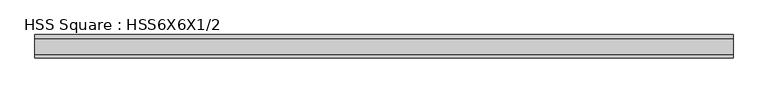
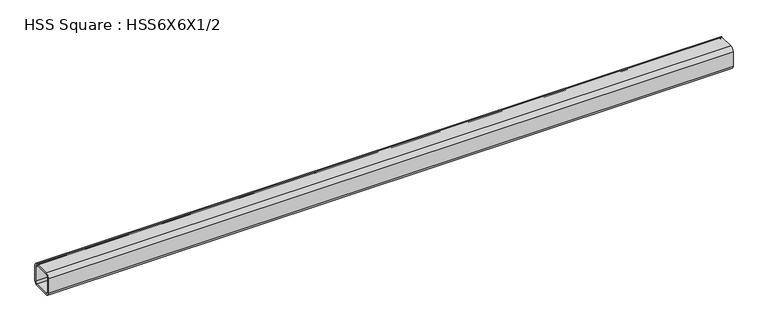
"""IFC4 building model written with IfcOpenShell, lengths in millimetres: member geometry, HSS Square : HSS6X6X1/2."""

import ifcopenshell
import ifcopenshell.guid

model = None  # the IFC model being written
_history = None  # IfcOwnerHistory: only IFC2X3 demands one
_inside = {}  # id of a spatial element -> (the spatial element, [elements in it])
_under = {}  # id of a project, library or spatial element -> (it, [spatial elements below it])
_declared = {}  # id of a project -> (the project, [libraries it declares])
_typed = {}  # id of a type object -> (the type object, [elements of that type])
_made_of = {}  # id of a material, layer set ... -> (it, [elements and type objects made of it])


def new_model(schema):
    """Start an empty IFC model of exactly this schema.

    Asked for "IFC4X3", IfcOpenShell would pick the latest addendum, in which some entities
    have other attributes; the version numbers below select the first issue.
    IFC2X3 requires an IfcOwnerHistory on every rooted entity: one is made here for all.
    """
    global model, _history
    if schema == "IFC4X3":
        model = ifcopenshell.file(schema_version=(4, 3, 0, 0))
    else:
        model = ifcopenshell.file(schema=schema)
    _inside.clear()
    _under.clear()
    _declared.clear()
    _typed.clear()
    _made_of.clear()
    _history = None
    if model.schema == "IFC2X3":
        org = make("IfcOrganization", Name="unknown")
        user = make(
            "IfcPersonAndOrganization",
            ThePerson=make("IfcPerson", FamilyName="unknown"),
            TheOrganization=org,
        )
        app = make(
            "IfcApplication",
            ApplicationDeveloper=org,
            Version="unknown",
            ApplicationFullName="unknown",
            ApplicationIdentifier="unknown",
        )
        _history = make(
            "IfcOwnerHistory",
            OwningUser=user,
            OwningApplication=app,
            ChangeAction="ADDED",
            CreationDate=0,
        )
    return model


def make(cls, **values):
    """One entity of the class cls with the attributes given. An attribute that is None is left unset."""
    return model.create_entity(
        cls, **{name: value for name, value in values.items() if value is not None}
    )


def rooted(cls, **values):
    """An entity with a GlobalId (a new one), such as an element, a storey or a relation."""
    return make(cls, GlobalId=ifcopenshell.guid.new(), OwnerHistory=_history, **values)


def si_unit(unit_type, name, prefix=None):
    """IfcSIUnit, for example si_unit("LENGTHUNIT", "METRE", prefix="MILLI")."""
    return make("IfcSIUnit", UnitType=unit_type, Prefix=prefix, Name=name)


def assignment(units):
    """IfcUnitAssignment: the units of a project."""
    return None if units is None else make("IfcUnitAssignment", Units=units)


def point(xyz):
    """IfcCartesianPoint."""
    return None if xyz is None else make("IfcCartesianPoint", Coordinates=xyz)


def direction(xyz):
    """IfcDirection."""
    return None if xyz is None else make("IfcDirection", DirectionRatios=xyz)


def frame(location, z_axis=None, x_axis=None):
    """IfcAxis2Placement3D, a coordinate frame: its origin and axes. An axis left out is left unset."""
    return make(
        "IfcAxis2Placement3D",
        Location=point(location),
        Axis=direction(z_axis),
        RefDirection=direction(x_axis),
    )


def frame_2d(location, x_axis=None):
    """IfcAxis2Placement2D, a coordinate frame in the plane: its origin and x axis."""
    return make(
        "IfcAxis2Placement2D", Location=point(location), RefDirection=direction(x_axis)
    )


def origin():
    """The frame at (0, 0, 0) with its axes left unset."""
    return frame((0.0, 0.0, 0.0))


def place(relative_to, where):
    """IfcLocalPlacement: puts the frame where relative to a parent placement (None: the world)."""
    return make(
        "IfcLocalPlacement", PlacementRelTo=relative_to, RelativePlacement=where
    )


def context(
    kind, dimensions, precision=None, world=None, true_north=None, identifier=None
):
    """IfcGeometricRepresentationContext, for example the 3D "Model" context."""
    return make(
        "IfcGeometricRepresentationContext",
        ContextIdentifier=identifier,
        ContextType=kind,
        CoordinateSpaceDimension=dimensions,
        Precision=precision,
        WorldCoordinateSystem=world,
        TrueNorth=true_north,
    )


def project(units=None, contexts=None):
    """IfcProject with its units and contexts."""
    return rooted(
        "IfcProject",
        Name="project",
        RepresentationContexts=contexts,
        UnitsInContext=assignment(units),
    )


def spatial(cls, under=None, at=None, **own):
    """A site, building, storey or space (cls), placed at a placement, below another one or the project."""
    s = rooted(cls, ObjectPlacement=at, **own)
    if under is not None:
        _under.setdefault(under.id(), (under, []))[1].append(s)
    return s


def polyline(points):
    """IfcPolyline through the points."""
    return make("IfcPolyline", Points=[point(p) for p in points])


def circle_curve(where, radius):
    """IfcCircle in the frame where."""
    return make("IfcCircle", Position=where, Radius=radius)


def trimmed(basis, trim1, trim2, sense, master):
    """IfcTrimmedCurve: the piece of a basis curve between two trims."""
    return make(
        "IfcTrimmedCurve",
        BasisCurve=basis,
        Trim1=trim1,
        Trim2=trim2,
        SenseAgreement=sense,
        MasterRepresentation=master,
    )


def segment(curve, same_sense, transition):
    """IfcCompositeCurveSegment."""
    return make(
        "IfcCompositeCurveSegment",
        Transition=transition,
        SameSense=same_sense,
        ParentCurve=curve,
    )


def composite_curve(segments, self_intersect=None):
    """IfcCompositeCurve: segments joined end to end."""
    return make("IfcCompositeCurve", Segments=segments, SelfIntersect=self_intersect)


def outline(outer, holes=None, kind="AREA"):
    """IfcArbitraryClosedProfileDef: a profile drawn as a closed curve; with holes, ...WithVoids."""
    if holes is None:
        return make("IfcArbitraryClosedProfileDef", ProfileType=kind, OuterCurve=outer)
    return make(
        "IfcArbitraryProfileDefWithVoids",
        ProfileType=kind,
        OuterCurve=outer,
        InnerCurves=holes,
    )


def extrude(swept, where, along, depth):
    """IfcExtrudedAreaSolid: the profile swept, set in the frame where, extruded along a direction by depth."""
    return make(
        "IfcExtrudedAreaSolid",
        SweptArea=swept,
        Position=where,
        ExtrudedDirection=direction(along),
        Depth=depth,
    )


def shape(context_of_items, identifier, shape_type, items):
    """IfcShapeRepresentation: the items that make up one representation, for example the "Body"."""
    return make(
        "IfcShapeRepresentation",
        ContextOfItems=context_of_items,
        RepresentationIdentifier=identifier,
        RepresentationType=shape_type,
        Items=items,
    )


def source(mapping_origin, context_of_items, identifier, shape_type, items):
    """IfcRepresentationMap: a shape defined once, which mapped items show again and again."""
    return make(
        "IfcRepresentationMap",
        MappingOrigin=mapping_origin,
        MappedRepresentation=shape(context_of_items, identifier, shape_type, items),
    )


def transform(
    local_origin,
    x_axis=None,
    y_axis=None,
    z_axis=None,
    scale=None,
    scale2=None,
    scale3=None,
    uniform=True,
):
    """IfcCartesianTransformationOperator3D, or its non-uniform kind. x_axis, y_axis, z_axis: its Axis1, 2, 3."""
    if uniform:
        return make(
            "IfcCartesianTransformationOperator3D",
            Axis1=direction(x_axis),
            Axis2=direction(y_axis),
            LocalOrigin=point(local_origin),
            Scale=scale,
            Axis3=direction(z_axis),
        )
    return make(
        "IfcCartesianTransformationOperator3DnonUniform",
        Axis1=direction(x_axis),
        Axis2=direction(y_axis),
        LocalOrigin=point(local_origin),
        Scale=scale,
        Axis3=direction(z_axis),
        Scale2=scale2,
        Scale3=scale3,
    )


def mapped(mapping_source, mapping_target):
    """IfcMappedItem: shows the shape of a source again, moved by a transform."""
    return make(
        "IfcMappedItem", MappingSource=mapping_source, MappingTarget=mapping_target
    )


def made_of(thing, what):
    """Note that an element or type object is made of a material, layer set ...; save() writes the relation."""
    if what is not None:
        _made_of.setdefault(what.id(), (what, []))[1].append(thing)
    return thing


def element(
    cls,
    number,
    at=None,
    inside=None,
    cuts=None,
    type_object=None,
    material=None,
    context=None,
    identifier="Body",
    shape_type=None,
    held_by="IfcProductDefinitionShape",
    body=None,
    shapes=None,
    **own,
):
    """One element of the class cls, such as IfcWall. Its Tag is "e" and its number.

    at: its placement. inside: the storey or other place that contains it. cuts: it is an
    opening in that element (IfcRelVoidsElement). A single representation is given by context,
    identifier, shape_type and body (its items); several are given by shapes. held_by: the class
    of the entity that holds the representations. save() writes the other relations.
    """
    e = rooted(cls, Tag="e%d" % number, ObjectPlacement=at, **own)
    if body is not None:
        shapes = [shape(context, identifier, shape_type, body)]
    if shapes is not None:
        e.Representation = make(held_by, Representations=shapes)
    if inside is not None:
        _inside.setdefault(inside.id(), (inside, []))[1].append(e)
    if cuts is not None:
        rooted(
            "IfcRelVoidsElement", RelatingBuildingElement=cuts, RelatedOpeningElement=e
        )
    if type_object is not None:
        _typed.setdefault(type_object.id(), (type_object, []))[1].append(e)
    return made_of(e, material)


def aggregate(whole, parts):
    """IfcRelAggregates: a whole, such as a stair, and the parts it consists of."""
    return rooted("IfcRelAggregates", RelatingObject=whole, RelatedObjects=parts)


def save(model, path):
    """Write the relations noted so far, then the file.

    IfcRelAggregates (storeys below a building ...), IfcRelContainedInSpatialStructure (elements
    in a storey), IfcRelDefinesByType, IfcRelAssociatesMaterial and IfcRelDeclares: one each for
    every whole, place, type object, material and project.
    """
    for whole, parts in _under.values():
        aggregate(whole, parts)
    for where, things in _inside.values():
        rooted(
            "IfcRelContainedInSpatialStructure",
            RelatedElements=things,
            RelatingStructure=where,
        )
    for kind, things in _typed.values():
        rooted("IfcRelDefinesByType", RelatedObjects=things, RelatingType=kind)
    for what, things in _made_of.values():
        rooted("IfcRelAssociatesMaterial", RelatedObjects=things, RelatingMaterial=what)
    for by, libraries in _declared.values():
        rooted("IfcRelDeclares", RelatingContext=by, RelatedDefinitions=libraries)
    model.write(path)


def hss_square_hss6x6x1_2_15cbbfaa(model_context):
    return source(origin(), model_context, "Body", "SweptSolid", [
        extrude(outline(composite_curve([segment(polyline([(76.2, 50.8), (76.2, -50.8)]), True, "CONTINUOUS"), segment(trimmed(circle_curve(frame_2d((50.8, -50.8)), 25.4), [point((76.2, -50.8))], [point((50.8, -76.2))], False, "CARTESIAN"), True, "CONTINUOUS"), segment(polyline([(50.8, -76.2), (-50.8, -76.2)]), True, "CONTINUOUS"), segment(trimmed(circle_curve(frame_2d((-50.8, -50.8)), 25.4), [point((-50.8, -76.2))], [point((-76.2, -50.8))], False, "CARTESIAN"), True, "CONTINUOUS"), segment(polyline([(-76.2, -50.8), (-76.2, 50.8)]), True, "CONTINUOUS"), segment(trimmed(circle_curve(frame_2d((-50.8, 50.8)), 25.4), [point((-76.2, 50.8))], [point((-50.8, 76.2))], False, "CARTESIAN"), True, "CONTINUOUS"), segment(polyline([(-50.8, 76.2), (50.8, 76.2)]), True, "CONTINUOUS"), segment(trimmed(circle_curve(frame_2d((50.8, 50.8)), 25.4), [point((50.8, 76.2))], [point((76.2, 50.8))], False, "CARTESIAN"), True, "CONTINUOUS")], self_intersect=False), holes=[composite_curve([segment(trimmed(circle_curve(frame_2d((-50.8, 50.8)), 12.7), [point((-50.8, 63.5))], [point((-63.5, 50.8))], True, "CARTESIAN"), True, "CONTINUOUS"), segment(polyline([(-63.5, 50.8), (-63.5, -50.8)]), True, "CONTINUOUS"), segment(trimmed(circle_curve(frame_2d((-50.8, -50.8)), 12.7), [point((-63.5, -50.8))], [point((-50.8, -63.5))], True, "CARTESIAN"), True, "CONTINUOUS"), segment(polyline([(-50.8, -63.5), (50.8, -63.5)]), True, "CONTINUOUS"), segment(trimmed(circle_curve(frame_2d((50.8, -50.8)), 12.7), [point((50.8, -63.5))], [point((63.5, -50.8))], True, "CARTESIAN"), True, "CONTINUOUS"), segment(polyline([(63.5, -50.8), (63.5, 50.8)]), True, "CONTINUOUS"), segment(trimmed(circle_curve(frame_2d((50.8, 50.8)), 12.7), [point((63.5, 50.8))], [point((50.8, 63.5))], True, "CARTESIAN"), True, "CONTINUOUS"), segment(polyline([(50.8, 63.5), (-50.8, 63.5)]), True, "CONTINUOUS")], self_intersect=False)]), frame((-2104.169756, 0.0, 0.0), z_axis=(1.0, 0.0, 0.0), x_axis=(0.0, 1.0, 0.0)), (0.0, 0.0, 1.0), 4524.6444945),
    ])


if __name__ == "__main__":
    model = new_model("IFC4")
    model_context = context("Model", 3, world=origin())
    ifc_project = project(units=[si_unit("LENGTHUNIT", "METRE", prefix="MILLI")], contexts=[model_context])
    site = spatial("IfcSite", under=ifc_project)
    building = spatial("IfcBuilding", under=site)
    placement = place(None, origin())
    hss_square_hss6x6x1_2_shape = hss_square_hss6x6x1_2_15cbbfaa(model_context)
    element("IfcMember", 1, ObjectType="HSS Square : HSS6X6X1/2", at=placement, inside=building, context=model_context, shape_type="MappedRepresentation", body=[
        mapped(hss_square_hss6x6x1_2_shape, transform((0.0, 0.0, 0.0), x_axis=(1.0, 0.0, 0.0), y_axis=(0.0, 1.0, 0.0), z_axis=(0.0, 0.0, 1.0))),
    ])
    save(model, "model.ifc")

# Revit data of these elements
# Type "HSS Square : HSS6X6X1/2"
#   Section Name Key = "HSS 6X6X1/2"
#   Assembly Code = "B10"
#   Width = 6.000"
#   Wall Nominal Thickness = 0.500"
#   Wall Design Thickness = 0.465"
#   Torsional Moment of Inertia = 81.10 in⁴
#   Torsional Modulus = 28.10 in³
#   Section Area = 9.74 in²
#   Plastic Modulus weak axis = 19.80 in³
#   Plastic Modulus strong axis = 19.80 in³
#   Outer Fillet = 1.000"
#   Nominal Weight = 35.24 lbf/ft
#   Moment of Inertia weak axis = 48.30 in⁴
#   Moment of Inertia strong axis = 48.30 in⁴
#   Inner Fillet = 0.500"
#   Height = 6.000"
#   Elastic Modulus weak axis = 16.10 in³
#   Elastic Modulus strong axis = 16.10 in³
#   Centroid Vertical = 3.000"
#   Centroid Horizontal = 3.000"
#   Length [instance default] = 5' - 0"
#   Structural Material [instance default] = Steel ASTM A500, Grade B, Rectangular and Square
#   Principal Axes Angle = 0
# Element 1 (IfcMember, "HSS Square : HSS6X6X1/2")
#   Structural Material = Steel ASTM A36
#   Materials on its faces: "Steel ASTM A36"
# Materials
#   "Steel ASTM A500, Grade B, Rectangular and Square": class "Metal", colour RGB 199 199 199, transparency 0, Description = "Carbon steel", Cost = 0
#   "Steel ASTM A36": class "Metal", colour RGB 199 199 199, transparency 0, Description = "Structural steel, ASTM A36 Grade B, mill finish", Cost = 0
